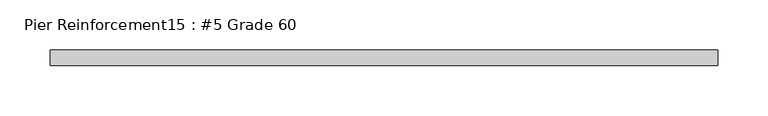
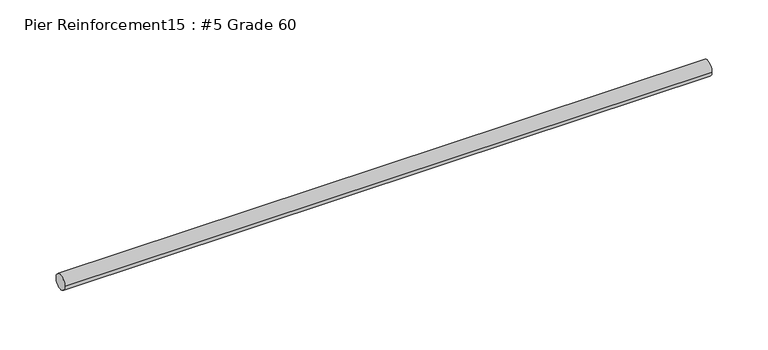
"""IFC4 building model written with IfcOpenShell, lengths in millimetres: proxy geometry, Pier Reinforcement15 : #5 Grade 60."""

from ifc_helpers import new_model, si_unit, point, frame, frame_2d, origin, place, context, project, spatial, circle_curve, trimmed, segment, composite_curve, outline, extrude, source, transform, mapped, element, save


def pier_reinforcement15_5_grade_60_756cefbf(model_context):
    return source(origin(), model_context, "Body", "SweptSolid", [
        extrude(outline(composite_curve([segment(trimmed(circle_curve(frame_2d((-531775.7413841, -55.5625)), 7.9375), [point((-531767.8038841, -55.5625))], [point((-531783.6788841, -55.5625))], False, "CARTESIAN"), True, "CONTINUOUS"), segment(trimmed(circle_curve(frame_2d((-531775.7413841, -55.5625)), 7.9375), [point((-531783.6788841, -55.5625))], [point((-531767.8038841, -55.5625))], False, "CARTESIAN"), True, "CONTINUOUS")], self_intersect=False)), frame((589567.2422365, 0.0, 0.0), z_axis=(1.0, 0.0, 0.0), x_axis=(0.0, 1.0, 0.0)), (0.0, 0.0, 1.0), 666.75),
    ])


if __name__ == "__main__":
    model = new_model("IFC4")
    model_context = context("Model", 3, world=origin())
    ifc_project = project(units=[si_unit("LENGTHUNIT", "METRE", prefix="MILLI")], contexts=[model_context])
    site = spatial("IfcSite", under=ifc_project)
    building = spatial("IfcBuilding", under=site)
    placement = place(None, origin())
    pier_reinforcement15_5_grade_60_shape = pier_reinforcement15_5_grade_60_756cefbf(model_context)
    element("IfcBuildingElementProxy", 1, Name="Pier Reinforcement15 : #5 Grade 60", ObjectType="Pier Reinforcement15 : #5 Grade 60", at=placement, inside=building, context=model_context, shape_type="MappedRepresentation", body=[
        mapped(pier_reinforcement15_5_grade_60_shape, transform((0.0, 0.0, 0.0), x_axis=(1.0, 0.0, 0.0), y_axis=(0.0, 1.0, 0.0), z_axis=(0.0, 0.0, 1.0))),
    ])
    save(model, "model.ifc")

# Revit data of these elements
# Element 1 (IfcBuildingElementProxy, "Pier Reinforcement15 : #5 Grade 60")
#   Materials on its faces: "#4 GR. 60 REINF. @ 16\" O.C. EW."
# Materials
#   "#4 GR. 60 REINF. @ 16\" O.C. EW.": class "Generic", colour RGB 84 83 81, transparency 0, Cost = 0
